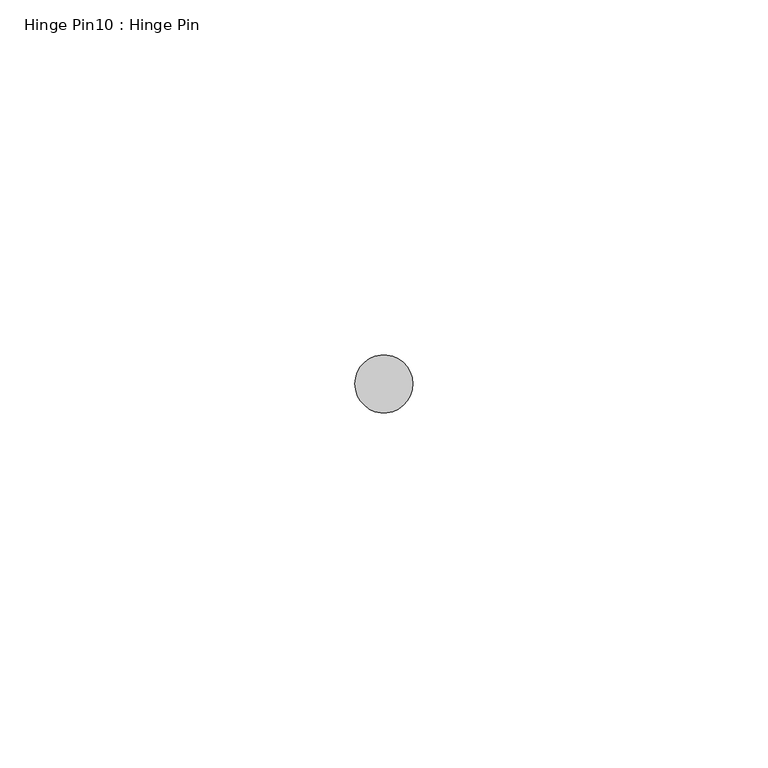
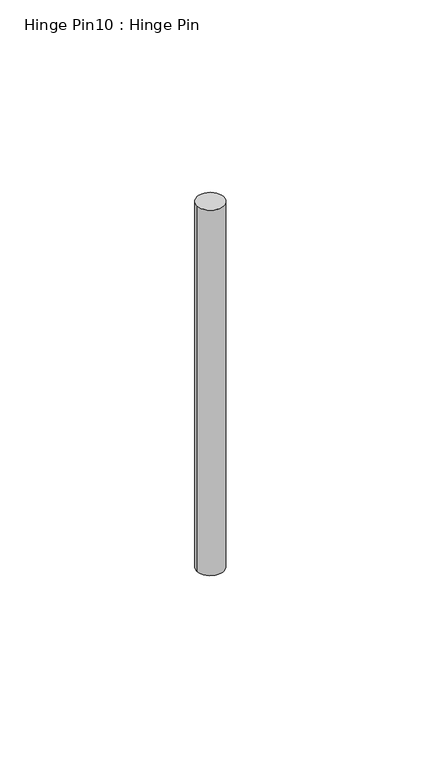
"""IFC4 building model written with IfcOpenShell, lengths in millimetres: proxy geometry, Hinge Pin10 : Hinge Pin."""

from ifc_helpers import new_model, si_unit, point, frame, frame_2d, origin, place, context, project, spatial, circle_curve, trimmed, segment, composite_curve, outline, extrude, source, transform, mapped, element, save


def hinge_pin10_hinge_pin_b100999e(model_context):
    return source(origin(), model_context, "Body", "SweptSolid", [
        extrude(outline(composite_curve([segment(trimmed(circle_curve(frame_2d((587319.1320739, -536310.3652841)), 4.0894), [point((587315.0426739, -536310.3652841))], [point((587323.2214739, -536310.3652841))], False, "CARTESIAN"), True, "CONTINUOUS"), segment(trimmed(circle_curve(frame_2d((587319.1320739, -536310.3652841)), 4.0894), [point((587323.2214739, -536310.3652841))], [point((587315.0426739, -536310.3652841))], False, "CARTESIAN"), True, "CONTINUOUS")], self_intersect=False)), frame((0.0, 0.0, 1941.3140625), z_axis=(0.0, 0.0, 1.0), x_axis=(1.0, 0.0, 0.0)), (0.0, 0.0, 1.0), 117.871875),
    ])


if __name__ == "__main__":
    model = new_model("IFC4")
    model_context = context("Model", 3, world=origin())
    ifc_project = project(units=[si_unit("LENGTHUNIT", "METRE", prefix="MILLI")], contexts=[model_context])
    site = spatial("IfcSite", under=ifc_project)
    building = spatial("IfcBuilding", under=site)
    placement = place(None, origin())
    hinge_pin10_hinge_pin_shape = hinge_pin10_hinge_pin_b100999e(model_context)
    element("IfcBuildingElementProxy", 1, Name="Hinge Pin10 : Hinge Pin", ObjectType="Hinge Pin10 : Hinge Pin", at=placement, inside=building, context=model_context, shape_type="MappedRepresentation", body=[
        mapped(hinge_pin10_hinge_pin_shape, transform((0.0, 0.0, 0.0), x_axis=(1.0, 0.0, 0.0), y_axis=(0.0, 1.0, 0.0), z_axis=(0.0, 0.0, 1.0))),
    ])
    save(model, "model.ifc")

# Revit data of these elements
# Element 1 (IfcBuildingElementProxy, "Hinge Pin10 : Hinge Pin")
#   Materials on its faces: "6\"X6\" WELD-ON STL BUTT HINGE"
# Materials
#   "6\"X6\" WELD-ON STL BUTT HINGE": class "Metal", colour RGB 189 187 185, transparency 0, Description = "Carbon steel", Cost = 0
